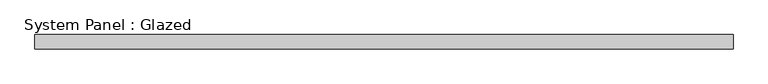
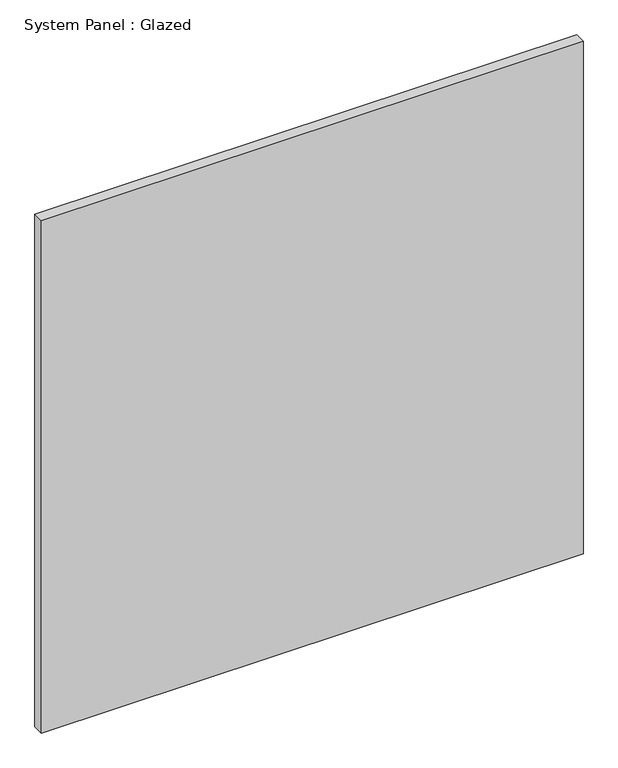
"""IFC4 building model written with IfcOpenShell, lengths in millimetres: plate geometry, System Panel : Glazed."""

import ifcopenshell
import ifcopenshell.guid

model = None  # the IFC model being written
_history = None  # IfcOwnerHistory: only IFC2X3 demands one
_inside = {}  # id of a spatial element -> (the spatial element, [elements in it])
_under = {}  # id of a project, library or spatial element -> (it, [spatial elements below it])
_declared = {}  # id of a project -> (the project, [libraries it declares])
_typed = {}  # id of a type object -> (the type object, [elements of that type])
_made_of = {}  # id of a material, layer set ... -> (it, [elements and type objects made of it])


def new_model(schema):
    """Start an empty IFC model of exactly this schema.

    Asked for "IFC4X3", IfcOpenShell would pick the latest addendum, in which some entities
    have other attributes; the version numbers below select the first issue.
    IFC2X3 requires an IfcOwnerHistory on every rooted entity: one is made here for all.
    """
    global model, _history
    if schema == "IFC4X3":
        model = ifcopenshell.file(schema_version=(4, 3, 0, 0))
    else:
        model = ifcopenshell.file(schema=schema)
    _inside.clear()
    _under.clear()
    _declared.clear()
    _typed.clear()
    _made_of.clear()
    _history = None
    if model.schema == "IFC2X3":
        org = make("IfcOrganization", Name="unknown")
        user = make(
            "IfcPersonAndOrganization",
            ThePerson=make("IfcPerson", FamilyName="unknown"),
            TheOrganization=org,
        )
        app = make(
            "IfcApplication",
            ApplicationDeveloper=org,
            Version="unknown",
            ApplicationFullName="unknown",
            ApplicationIdentifier="unknown",
        )
        _history = make(
            "IfcOwnerHistory",
            OwningUser=user,
            OwningApplication=app,
            ChangeAction="ADDED",
            CreationDate=0,
        )
    return model


def make(cls, **values):
    """One entity of the class cls with the attributes given. An attribute that is None is left unset."""
    return model.create_entity(
        cls, **{name: value for name, value in values.items() if value is not None}
    )


def rooted(cls, **values):
    """An entity with a GlobalId (a new one), such as an element, a storey or a relation."""
    return make(cls, GlobalId=ifcopenshell.guid.new(), OwnerHistory=_history, **values)


def si_unit(unit_type, name, prefix=None):
    """IfcSIUnit, for example si_unit("LENGTHUNIT", "METRE", prefix="MILLI")."""
    return make("IfcSIUnit", UnitType=unit_type, Prefix=prefix, Name=name)


def assignment(units):
    """IfcUnitAssignment: the units of a project."""
    return None if units is None else make("IfcUnitAssignment", Units=units)


def point(xyz):
    """IfcCartesianPoint."""
    return None if xyz is None else make("IfcCartesianPoint", Coordinates=xyz)


def direction(xyz):
    """IfcDirection."""
    return None if xyz is None else make("IfcDirection", DirectionRatios=xyz)


def frame(location, z_axis=None, x_axis=None):
    """IfcAxis2Placement3D, a coordinate frame: its origin and axes. An axis left out is left unset."""
    return make(
        "IfcAxis2Placement3D",
        Location=point(location),
        Axis=direction(z_axis),
        RefDirection=direction(x_axis),
    )


def origin():
    """The frame at (0, 0, 0) with its axes left unset."""
    return frame((0.0, 0.0, 0.0))


def origin_with_axes():
    """The frame at (0, 0, 0) with the z axis (0, 0, 1) and the x axis (1, 0, 0) written out."""
    return frame((0.0, 0.0, 0.0), z_axis=(0.0, 0.0, 1.0), x_axis=(1.0, 0.0, 0.0))


def place(relative_to, where):
    """IfcLocalPlacement: puts the frame where relative to a parent placement (None: the world)."""
    return make(
        "IfcLocalPlacement", PlacementRelTo=relative_to, RelativePlacement=where
    )


def context(
    kind, dimensions, precision=None, world=None, true_north=None, identifier=None
):
    """IfcGeometricRepresentationContext, for example the 3D "Model" context."""
    return make(
        "IfcGeometricRepresentationContext",
        ContextIdentifier=identifier,
        ContextType=kind,
        CoordinateSpaceDimension=dimensions,
        Precision=precision,
        WorldCoordinateSystem=world,
        TrueNorth=true_north,
    )


def project(units=None, contexts=None):
    """IfcProject with its units and contexts."""
    return rooted(
        "IfcProject",
        Name="project",
        RepresentationContexts=contexts,
        UnitsInContext=assignment(units),
    )


def spatial(cls, under=None, at=None, **own):
    """A site, building, storey or space (cls), placed at a placement, below another one or the project."""
    s = rooted(cls, ObjectPlacement=at, **own)
    if under is not None:
        _under.setdefault(under.id(), (under, []))[1].append(s)
    return s


def polyline(points):
    """IfcPolyline through the points."""
    return make("IfcPolyline", Points=[point(p) for p in points])


def outline(outer, holes=None, kind="AREA"):
    """IfcArbitraryClosedProfileDef: a profile drawn as a closed curve; with holes, ...WithVoids."""
    if holes is None:
        return make("IfcArbitraryClosedProfileDef", ProfileType=kind, OuterCurve=outer)
    return make(
        "IfcArbitraryProfileDefWithVoids",
        ProfileType=kind,
        OuterCurve=outer,
        InnerCurves=holes,
    )


def extrude(swept, where, along, depth):
    """IfcExtrudedAreaSolid: the profile swept, set in the frame where, extruded along a direction by depth."""
    return make(
        "IfcExtrudedAreaSolid",
        SweptArea=swept,
        Position=where,
        ExtrudedDirection=direction(along),
        Depth=depth,
    )


def shape(context_of_items, identifier, shape_type, items):
    """IfcShapeRepresentation: the items that make up one representation, for example the "Body"."""
    return make(
        "IfcShapeRepresentation",
        ContextOfItems=context_of_items,
        RepresentationIdentifier=identifier,
        RepresentationType=shape_type,
        Items=items,
    )


def source(mapping_origin, context_of_items, identifier, shape_type, items):
    """IfcRepresentationMap: a shape defined once, which mapped items show again and again."""
    return make(
        "IfcRepresentationMap",
        MappingOrigin=mapping_origin,
        MappedRepresentation=shape(context_of_items, identifier, shape_type, items),
    )


def transform(
    local_origin,
    x_axis=None,
    y_axis=None,
    z_axis=None,
    scale=None,
    scale2=None,
    scale3=None,
    uniform=True,
):
    """IfcCartesianTransformationOperator3D, or its non-uniform kind. x_axis, y_axis, z_axis: its Axis1, 2, 3."""
    if uniform:
        return make(
            "IfcCartesianTransformationOperator3D",
            Axis1=direction(x_axis),
            Axis2=direction(y_axis),
            LocalOrigin=point(local_origin),
            Scale=scale,
            Axis3=direction(z_axis),
        )
    return make(
        "IfcCartesianTransformationOperator3DnonUniform",
        Axis1=direction(x_axis),
        Axis2=direction(y_axis),
        LocalOrigin=point(local_origin),
        Scale=scale,
        Axis3=direction(z_axis),
        Scale2=scale2,
        Scale3=scale3,
    )


def mapped(mapping_source, mapping_target):
    """IfcMappedItem: shows the shape of a source again, moved by a transform."""
    return make(
        "IfcMappedItem", MappingSource=mapping_source, MappingTarget=mapping_target
    )


def made_of(thing, what):
    """Note that an element or type object is made of a material, layer set ...; save() writes the relation."""
    if what is not None:
        _made_of.setdefault(what.id(), (what, []))[1].append(thing)
    return thing


def element(
    cls,
    number,
    at=None,
    inside=None,
    cuts=None,
    type_object=None,
    material=None,
    context=None,
    identifier="Body",
    shape_type=None,
    held_by="IfcProductDefinitionShape",
    body=None,
    shapes=None,
    **own,
):
    """One element of the class cls, such as IfcWall. Its Tag is "e" and its number.

    at: its placement. inside: the storey or other place that contains it. cuts: it is an
    opening in that element (IfcRelVoidsElement). A single representation is given by context,
    identifier, shape_type and body (its items); several are given by shapes. held_by: the class
    of the entity that holds the representations. save() writes the other relations.
    """
    e = rooted(cls, Tag="e%d" % number, ObjectPlacement=at, **own)
    if body is not None:
        shapes = [shape(context, identifier, shape_type, body)]
    if shapes is not None:
        e.Representation = make(held_by, Representations=shapes)
    if inside is not None:
        _inside.setdefault(inside.id(), (inside, []))[1].append(e)
    if cuts is not None:
        rooted(
            "IfcRelVoidsElement", RelatingBuildingElement=cuts, RelatedOpeningElement=e
        )
    if type_object is not None:
        _typed.setdefault(type_object.id(), (type_object, []))[1].append(e)
    return made_of(e, material)


def aggregate(whole, parts):
    """IfcRelAggregates: a whole, such as a stair, and the parts it consists of."""
    return rooted("IfcRelAggregates", RelatingObject=whole, RelatedObjects=parts)


def save(model, path):
    """Write the relations noted so far, then the file.

    IfcRelAggregates (storeys below a building ...), IfcRelContainedInSpatialStructure (elements
    in a storey), IfcRelDefinesByType, IfcRelAssociatesMaterial and IfcRelDeclares: one each for
    every whole, place, type object, material and project.
    """
    for whole, parts in _under.values():
        aggregate(whole, parts)
    for where, things in _inside.values():
        rooted(
            "IfcRelContainedInSpatialStructure",
            RelatedElements=things,
            RelatingStructure=where,
        )
    for kind, things in _typed.values():
        rooted("IfcRelDefinesByType", RelatedObjects=things, RelatingType=kind)
    for what, things in _made_of.values():
        rooted("IfcRelAssociatesMaterial", RelatedObjects=things, RelatingMaterial=what)
    for by, libraries in _declared.values():
        rooted("IfcRelDeclares", RelatingContext=by, RelatedDefinitions=libraries)
    model.write(path)


def system_panel_glazed_84cf4e26(model_context):
    return source(origin(), model_context, "Body", "SweptSolid", [
        extrude(outline(polyline([(609.6, 19.05), (-609.6, 19.05), (-609.6, 44.45), (609.6, 44.45), (609.6, 19.05)])), origin_with_axes(), (0.0, 0.0, 1.0), 1219.2),
    ])


if __name__ == "__main__":
    model = new_model("IFC4")
    model_context = context("Model", 3, world=origin())
    ifc_project = project(units=[si_unit("LENGTHUNIT", "METRE", prefix="MILLI")], contexts=[model_context])
    site = spatial("IfcSite", under=ifc_project)
    building = spatial("IfcBuilding", under=site)
    placement = place(None, origin())
    system_panel_glazed_shape = system_panel_glazed_84cf4e26(model_context)
    element("IfcPlate", 1, ObjectType="System Panel : Glazed", at=placement, inside=building, context=model_context, shape_type="MappedRepresentation", body=[
        mapped(system_panel_glazed_shape, transform((0.0, 0.0, 0.0), x_axis=(1.0, 0.0, 0.0), y_axis=(0.0, 1.0, 0.0), z_axis=(0.0, 0.0, 1.0))),
    ])
    save(model, "model.ifc")

# Revit data of these elements
# Element 1 (IfcPlate, "System Panel : Glazed")
#   Materials on its faces: "Glass"
# Materials
#   "Glass": class "Glass", colour RGB 0 128 192, transparency 0.75
